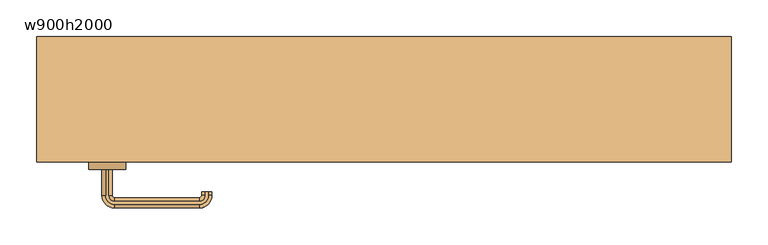
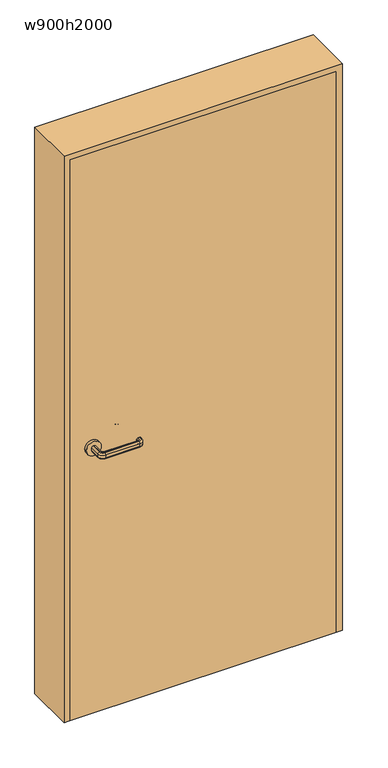
"""IFC4 building model written with IfcOpenShell, lengths in millimetres: door geometry, 片開き : w900h2000."""

from ifc_helpers import new_model, si_unit, point, frame, frame_2d, origin, origin_with_axes, place, context, project, spatial, polyline, circle_curve, ellipse_curve, trimmed, segment, composite_curve, outline, extrude, source, transform, mapped, element, save
from ifc_brep_helpers import plane_surface, cylinder_surface, revolved_surface, advanced_brep


def w900h2000_4bf1bc26(model_context):
    return source(origin(), model_context, "Body", "SolidModel", [
        advanced_brep(
        [(-377.0, -95.0, 960.0), (-373.0, -95.0, 960.0), (-368.0, -95.0, 955.0), (-368.0, -95.0, 945.0477623), (-373.0, -95.0, 940.0477623), (-377.0, -95.0, 940.0477623), (-382.0, -95.0, 945.0477623), (-382.0, -95.0, 955.0), (-382.0, -130.0, 955.0), (-377.0, -130.0, 960.0), (-382.0, -130.0, 945.0477623), (-377.0, -130.0, 940.0477623), (-373.0, -130.0, 940.0477623), (-365.0, -138.0, 940.0477623), (-250.0, -138.0, 940.0477623), (-242.0, -130.0, 940.0477623), (-242.0, -125.0, 940.0477623), (-238.0, -125.0, 940.0477623), (-238.0, -130.0, 940.0477623), (-250.0, -142.0, 940.0477623), (-365.0, -142.0, 940.0477623), (-368.0, -130.0, 945.0477623), (-368.0, -130.0, 955.0), (-373.0, -130.0, 960.0), (-365.0, -142.0, 960.0), (-250.0, -142.0, 960.0), (-238.0, -130.0, 960.0), (-238.0, -125.0, 960.0), (-242.0, -125.0, 960.0), (-242.0, -130.0, 960.0), (-250.0, -138.0, 960.0), (-365.0, -138.0, 960.0), (-365.0, -147.0, 955.0), (-365.0, -147.0, 945.0477623), (-365.0, -133.0, 945.0477623), (-365.0, -133.0, 955.0), (-250.0, -147.0, 955.0), (-250.0, -147.0, 945.0477623), (-250.0, -133.0, 945.0477623), (-250.0, -133.0, 955.0), (-233.0, -130.0, 955.0), (-233.0, -130.0, 945.0477623), (-247.0, -130.0, 945.0477623), (-247.0, -130.0, 955.0), (-233.0, -125.0, 955.0), (-233.0, -125.0, 945.0477623), (-247.0, -125.0, 945.0477623), (-247.0, -125.0, 955.0)],
        [
            (0, 1),
            (1, 2, circle_curve(frame((-373.0, -95.0, 955.0), z_axis=(0.0, 1.0, 0.0), x_axis=(-1.0, 0.0, 0.0)), 5.0)),
            (2, 3),
            (3, 4, circle_curve(frame((-373.0, -95.0, 945.0477623), z_axis=(0.0, 1.0, 0.0), x_axis=(-1.0, 0.0, 0.0)), 5.0)),
            (4, 5),
            (5, 6, circle_curve(frame((-377.0, -95.0, 945.0477623), z_axis=(0.0, 1.0, 0.0), x_axis=(-1.0, 0.0, 0.0)), 5.0)),
            (6, 7),
            (7, 0, circle_curve(frame((-377.0, -95.0, 955.0), z_axis=(0.0, 1.0, 0.0), x_axis=(-1.0, 0.0, 0.0)), 5.0)),
            (7, 8),
            (8, 9, circle_curve(frame((-377.0, -130.0, 955.0), z_axis=(0.0, 1.0, 0.0), x_axis=(-1.0, 0.0, 0.0)), 5.0)),
            (9, 0),
            (6, 10),
            (10, 8),
            (5, 11),
            (11, 10, circle_curve(frame((-377.0, -130.0, 945.0477623), z_axis=(0.0, 1.0, 0.0), x_axis=(-1.0, 0.0, 0.0)), 5.0)),
            (4, 12),
            (12, 13, circle_curve(frame((-365.0, -130.0, 940.0477623), z_axis=(0.0, 0.0, 1.0), x_axis=(-1.0, 0.0, 0.0)), 8.0)),
            (13, 14),
            (14, 15, circle_curve(frame((-250.0, -130.0, 940.0477623), z_axis=(0.0, 0.0, 1.0), x_axis=(0.0, -1.0, 0.0)), 8.0)),
            (15, 16),
            (16, 17),
            (17, 18),
            (18, 19, circle_curve(frame((-250.0, -130.0, 940.0477623), z_axis=(0.0, 0.0, -1.0), x_axis=(0.0, -1.0, 0.0)), 12.0)),
            (19, 20),
            (20, 11, circle_curve(frame((-365.0, -130.0, 940.0477623), z_axis=(0.0, 0.0, -1.0), x_axis=(-1.0, 0.0, 0.0)), 12.0)),
            (3, 21),
            (21, 12, circle_curve(frame((-373.0, -130.0, 945.0477623), z_axis=(0.0, 1.0, 0.0), x_axis=(-1.0, 0.0, 0.0)), 5.0)),
            (2, 22),
            (22, 21),
            (1, 23),
            (23, 22, circle_curve(frame((-373.0, -130.0, 955.0), z_axis=(0.0, 1.0, 0.0), x_axis=(-1.0, 0.0, 0.0)), 5.0)),
            (9, 24, circle_curve(frame((-365.0, -130.0, 960.0), z_axis=(0.0, 0.0, 1.0), x_axis=(-1.0, 0.0, 0.0)), 12.0)),
            (24, 25),
            (25, 26, circle_curve(frame((-250.0, -130.0, 960.0), z_axis=(0.0, 0.0, 1.0), x_axis=(0.0, -1.0, 0.0)), 12.0)),
            (26, 27),
            (27, 28),
            (28, 29),
            (29, 30, circle_curve(frame((-250.0, -130.0, 960.0), z_axis=(0.0, 0.0, -1.0), x_axis=(0.0, -1.0, 0.0)), 8.0)),
            (30, 31),
            (31, 23, circle_curve(frame((-365.0, -130.0, 960.0), z_axis=(0.0, 0.0, -1.0), x_axis=(-1.0, 0.0, 0.0)), 8.0)),
            (32, 24, circle_curve(frame((-365.0, -142.0, 955.0), z_axis=(-1.0, 0.0, 0.0), x_axis=(0.0, -1.0, 0.0)), 5.0)),
            (8, 32, circle_curve(frame((-365.0, -130.0, 955.0), z_axis=(0.0, 0.0, 1.0), x_axis=(-1.0, 0.0, 0.0)), 17.0)),
            (33, 32),
            (10, 33, circle_curve(frame((-365.0, -130.0, 945.0477623), z_axis=(0.0, 0.0, 1.0), x_axis=(-1.0, 0.0, 0.0)), 17.0)),
            (20, 33, circle_curve(frame((-365.0, -142.0, 945.0477623), z_axis=(-1.0, 0.0, 0.0), x_axis=(0.0, -1.0, 0.0)), 5.0)),
            (34, 13, circle_curve(frame((-365.0, -138.0, 945.0477623), z_axis=(-1.0, 0.0, 0.0), x_axis=(0.0, -1.0, 0.0)), 5.0)),
            (21, 34, circle_curve(frame((-365.0, -130.0, 945.0477623), z_axis=(0.0, 0.0, 1.0), x_axis=(-1.0, 0.0, 0.0)), 3.0)),
            (35, 34),
            (22, 35, circle_curve(frame((-365.0, -130.0, 955.0), z_axis=(0.0, 0.0, 1.0), x_axis=(-1.0, 0.0, 0.0)), 3.0)),
            (31, 35, circle_curve(frame((-365.0, -138.0, 955.0), z_axis=(-1.0, 0.0, 0.0), x_axis=(0.0, -1.0, 0.0)), 5.0)),
            (32, 36),
            (36, 25, circle_curve(frame((-250.0, -142.0, 955.0), z_axis=(-1.0, 0.0, 0.0), x_axis=(0.0, -1.0, 0.0)), 5.0)),
            (33, 37),
            (37, 36),
            (19, 37, circle_curve(frame((-250.0, -142.0, 945.0477623), z_axis=(-1.0, 0.0, 0.0), x_axis=(0.0, -1.0, 0.0)), 5.0)),
            (34, 38),
            (38, 14, circle_curve(frame((-250.0, -138.0, 945.0477623), z_axis=(-1.0, 0.0, 0.0), x_axis=(0.0, -1.0, 0.0)), 5.0)),
            (35, 39),
            (39, 38),
            (30, 39, circle_curve(frame((-250.0, -138.0, 955.0), z_axis=(-1.0, 0.0, 0.0), x_axis=(0.0, -1.0, 0.0)), 5.0)),
            (40, 26, circle_curve(frame((-238.0, -130.0, 955.0), z_axis=(0.0, -1.0, 0.0), x_axis=(1.0, 0.0, 0.0)), 5.0)),
            (36, 40, circle_curve(frame((-250.0, -130.0, 955.0), z_axis=(0.0, 0.0, 1.0), x_axis=(0.0, -1.0, 0.0)), 17.0)),
            (41, 40),
            (37, 41, circle_curve(frame((-250.0, -130.0, 945.0477623), z_axis=(0.0, 0.0, 1.0), x_axis=(0.0, -1.0, 0.0)), 17.0)),
            (18, 41, circle_curve(frame((-238.0, -130.0, 945.0477623), z_axis=(0.0, -1.0, 0.0), x_axis=(1.0, 0.0, 0.0)), 5.0)),
            (42, 15, circle_curve(frame((-242.0, -130.0, 945.0477623), z_axis=(0.0, -1.0, 0.0), x_axis=(1.0, 0.0, 0.0)), 5.0)),
            (38, 42, circle_curve(frame((-250.0, -130.0, 945.0477623), z_axis=(0.0, 0.0, 1.0), x_axis=(0.0, -1.0, 0.0)), 3.0)),
            (43, 42),
            (39, 43, circle_curve(frame((-250.0, -130.0, 955.0), z_axis=(0.0, 0.0, 1.0), x_axis=(0.0, -1.0, 0.0)), 3.0)),
            (29, 43, circle_curve(frame((-242.0, -130.0, 955.0), z_axis=(0.0, -1.0, 0.0), x_axis=(1.0, 0.0, 0.0)), 5.0)),
            (27, 44, circle_curve(frame((-238.0, -125.0, 955.0), z_axis=(0.0, 1.0, 0.0), x_axis=(1.0, 0.0, 0.0)), 5.0)),
            (44, 45),
            (45, 17, circle_curve(frame((-238.0, -125.0, 945.0477623), z_axis=(0.0, 1.0, 0.0), x_axis=(1.0, 0.0, 0.0)), 5.0)),
            (16, 46, circle_curve(frame((-242.0, -125.0, 945.0477623), z_axis=(0.0, 1.0, 0.0), x_axis=(1.0, 0.0, 0.0)), 5.0)),
            (46, 47),
            (47, 28, circle_curve(frame((-242.0, -125.0, 955.0), z_axis=(0.0, 1.0, 0.0), x_axis=(1.0, 0.0, 0.0)), 5.0)),
            (40, 44),
            (41, 45),
            (42, 46),
            (43, 47),
        ],
        [
            plane_surface(frame((-385.198039, -95.0, 950.0), z_axis=(0.0, 1.0, 0.0), x_axis=(0.0, 0.0, 1.0))),
            cylinder_surface(frame((-377.0, -95.0, 955.0), z_axis=(0.0, 1.0, 0.0), x_axis=(-1.0, 0.0, 0.0)), 5.0),
            plane_surface(frame((-382.0, -95.0, 955.0), z_axis=(-1.0, 0.0, 0.0), x_axis=(0.0, -1.0, 0.0))),
            cylinder_surface(frame((-377.0, -95.0, 945.0477623), z_axis=(0.0, 1.0, 0.0), x_axis=(-1.0, 0.0, 0.0)), 5.0),
            plane_surface(frame((-377.0, -95.0, 940.0477623), z_axis=(0.0, 0.0, -1.0), x_axis=(0.0, -1.0, 0.0))),
            cylinder_surface(frame((-373.0, -95.0, 945.0477623), z_axis=(0.0, 1.0, 0.0), x_axis=(-1.0, 0.0, 0.0)), 5.0),
            plane_surface(frame((-368.0, -95.0, 945.0477623), z_axis=(1.0, 0.0, 0.0), x_axis=(0.0, -1.0, 0.0))),
            cylinder_surface(frame((-373.0, -95.0, 955.0), z_axis=(0.0, 1.0, 0.0), x_axis=(-1.0, 0.0, 0.0)), 5.0),
            plane_surface(frame((-373.0, -95.0, 960.0), z_axis=(0.0, 0.0, 1.0), x_axis=(0.0, -1.0, 0.0))),
            revolved_surface(trimmed(ellipse_curve(frame((-377.0, -130.0, 955.0), z_axis=(0.0, -1.0, 0.0), x_axis=(-1.0, 0.0, 0.0)), 5.0, 5.0), [point((-377.0, -130.0, 960.0))], [point((-382.0, -130.0, 955.0))], True, "CARTESIAN"), (-365.0, -130.0, 950.0), (0.0, 0.0, -1.0)),
            cylinder_surface(frame((-365.0, -130.0, 950.0), z_axis=(0.0, 0.0, -1.0), x_axis=(-1.0, 0.0, 0.0)), 17.0),
            revolved_surface(trimmed(ellipse_curve(frame((-377.0, -130.0, 945.0477623), z_axis=(0.0, -1.0, 0.0), x_axis=(-1.0, 0.0, 0.0)), 5.0, 5.0), [point((-382.0, -130.0, 945.0477623))], [point((-377.0, -130.0, 940.0477623))], True, "CARTESIAN"), (-365.0, -130.0, 950.0), (0.0, 0.0, -1.0)),
            revolved_surface(trimmed(ellipse_curve(frame((-373.0, -130.0, 945.0477623), z_axis=(0.0, -1.0, 0.0), x_axis=(-1.0, 0.0, 0.0)), 5.0, 5.0), [point((-373.0, -130.0, 940.0477623))], [point((-368.0, -130.0, 945.0477623))], True, "CARTESIAN"), (-365.0, -130.0, 950.0), (0.0, 0.0, -1.0)),
            revolved_surface(polyline([(-368.0, -130.0, 945.0477623), (-368.0, -130.0, 955.0)]), (-365.0, -130.0, 950.0), (0.0, 0.0, -1.0)),
            revolved_surface(trimmed(ellipse_curve(frame((-373.0, -130.0, 955.0), z_axis=(0.0, -1.0, 0.0), x_axis=(-1.0, 0.0, 0.0)), 5.0, 5.0), [point((-368.0, -130.0, 955.0))], [point((-373.0, -130.0, 960.0))], True, "CARTESIAN"), (-365.0, -130.0, 950.0), (0.0, 0.0, -1.0)),
            cylinder_surface(frame((-365.0, -142.0, 955.0), z_axis=(-1.0, 0.0, 0.0), x_axis=(0.0, -1.0, 0.0)), 5.0),
            plane_surface(frame((-365.0, -147.0, 955.0), z_axis=(0.0, -1.0, 0.0), x_axis=(1.0, 0.0, 0.0))),
            cylinder_surface(frame((-365.0, -142.0, 945.0477623), z_axis=(-1.0, 0.0, 0.0), x_axis=(0.0, -1.0, 0.0)), 5.0),
            cylinder_surface(frame((-365.0, -138.0, 945.0477623), z_axis=(-1.0, 0.0, 0.0), x_axis=(0.0, -1.0, 0.0)), 5.0),
            plane_surface(frame((-365.0, -133.0, 945.0477623), z_axis=(0.0, 1.0, 0.0), x_axis=(1.0, 0.0, 0.0))),
            cylinder_surface(frame((-365.0, -138.0, 955.0), z_axis=(-1.0, 0.0, 0.0), x_axis=(0.0, -1.0, 0.0)), 5.0),
            revolved_surface(trimmed(ellipse_curve(frame((-250.0, -142.0, 955.0), z_axis=(1.0, 0.0, 0.0), x_axis=(0.0, -1.0, 0.0)), 5.0, 5.0), [point((-250.0, -142.0, 960.0))], [point((-250.0, -147.0, 955.0))], True, "CARTESIAN"), (-250.0, -130.0, 950.0), (0.0, 0.0, -1.0)),
            cylinder_surface(frame((-250.0, -130.0, 950.0), z_axis=(0.0, 0.0, -1.0), x_axis=(0.0, -1.0, 0.0)), 17.0),
            revolved_surface(trimmed(ellipse_curve(frame((-250.0, -142.0, 945.0477623), z_axis=(1.0, 0.0, 0.0), x_axis=(0.0, -1.0, 0.0)), 5.0, 5.0), [point((-250.0, -147.0, 945.0477623))], [point((-250.0, -142.0, 940.0477623))], True, "CARTESIAN"), (-250.0, -130.0, 950.0), (0.0, 0.0, -1.0)),
            revolved_surface(trimmed(ellipse_curve(frame((-250.0, -138.0, 945.0477623), z_axis=(1.0, 0.0, 0.0), x_axis=(0.0, -1.0, 0.0)), 5.0, 5.0), [point((-250.0, -138.0, 940.0477623))], [point((-250.0, -133.0, 945.0477623))], True, "CARTESIAN"), (-250.0, -130.0, 950.0), (0.0, 0.0, -1.0)),
            revolved_surface(polyline([(-250.0, -133.0, 945.0477623), (-250.0, -133.0, 955.0)]), (-250.0, -130.0, 950.0), (0.0, 0.0, -1.0)),
            revolved_surface(trimmed(ellipse_curve(frame((-250.0, -138.0, 955.0), z_axis=(1.0, 0.0, 0.0), x_axis=(0.0, -1.0, 0.0)), 5.0, 5.0), [point((-250.0, -133.0, 955.0))], [point((-250.0, -138.0, 960.0))], True, "CARTESIAN"), (-250.0, -130.0, 950.0), (0.0, 0.0, -1.0)),
            plane_surface(frame((-250.198039, -125.0, 950.0), z_axis=(0.0, 1.0, 0.0), x_axis=(0.0, 0.0, -1.0))),
            cylinder_surface(frame((-238.0, -130.0, 955.0), z_axis=(0.0, -1.0, 0.0), x_axis=(1.0, 0.0, 0.0)), 5.0),
            plane_surface(frame((-233.0, -130.0, 955.0), z_axis=(1.0, 0.0, 0.0), x_axis=(0.0, 1.0, 0.0))),
            cylinder_surface(frame((-238.0, -130.0, 945.0477623), z_axis=(0.0, -1.0, 0.0), x_axis=(1.0, 0.0, 0.0)), 5.0),
            cylinder_surface(frame((-242.0, -130.0, 945.0477623), z_axis=(0.0, -1.0, 0.0), x_axis=(1.0, 0.0, 0.0)), 5.0),
            plane_surface(frame((-247.0, -130.0, 945.0477623), z_axis=(-1.0, 0.0, 0.0), x_axis=(0.0, 1.0, 0.0))),
            cylinder_surface(frame((-242.0, -130.0, 955.0), z_axis=(0.0, -1.0, 0.0), x_axis=(1.0, 0.0, 0.0)), 5.0),
        ],
        [
            (0, [[1, 2, 3, 4, 5, 6, 7, 8]]),
            (1, [[9, 10, 11, -8]]),
            (2, [[12, 13, -9, -7]]),
            (3, [[14, 15, -12, -6]]),
            (4, [[16, 17, 18, 19, 20, 21, 22, 23, 24, 25, -14, -5]]),
            (5, [[26, 27, -16, -4]]),
            (6, [[28, 29, -26, -3]]),
            (7, [[30, 31, -28, -2]]),
            (8, [[-11, 32, 33, 34, 35, 36, 37, 38, 39, 40, -30, -1]]),
            (9, [[41, -32, -10, 42]]),
            (10, [[43, -42, -13, 44]]),
            (11, [[45, -44, -15, -25]]),
            (12, [[46, -17, -27, 47]]),
            (13, [[48, -47, -29, 49]]),
            (14, [[50, -49, -31, -40]]),
            (15, [[51, 52, -33, -41]]),
            (16, [[53, 54, -51, -43]]),
            (17, [[-24, 55, -53, -45]]),
            (18, [[56, 57, -18, -46]]),
            (19, [[58, 59, -56, -48]]),
            (20, [[-39, 60, -58, -50]]),
            (21, [[61, -34, -52, 62]]),
            (22, [[63, -62, -54, 64]]),
            (23, [[65, -64, -55, -23]]),
            (24, [[66, -19, -57, 67]]),
            (25, [[68, -67, -59, 69]]),
            (26, [[70, -69, -60, -38]]),
            (27, [[71, 72, 73, -21, 74, 75, 76, -36]]),
            (28, [[77, -71, -35, -61]]),
            (29, [[78, -72, -77, -63]]),
            (30, [[-22, -73, -78, -65]]),
            (31, [[79, -74, -20, -66]]),
            (32, [[80, -75, -79, -68]]),
            (33, [[-37, -76, -80, -70]]),
        ],
    ),
        advanced_brep(
        [(-373.0, -50.0, 940.0), (-368.0, -50.0, 945.0), (-368.0, -50.0, 955.0), (-373.0, -50.0, 960.0), (-377.0, -50.0, 960.0), (-382.0, -50.0, 955.0), (-382.0, -50.0, 945.0), (-377.0, -50.0, 940.0), (-377.0, -15.0, 940.0), (-365.0, -3.0, 940.0), (-250.0, -3.0, 940.0), (-238.0, -15.0, 940.0), (-238.0, -20.0, 940.0), (-242.0, -20.0, 940.0), (-242.0, -15.0, 940.0), (-250.0, -7.0, 940.0), (-365.0, -7.0, 940.0), (-373.0, -15.0, 940.0), (-382.0, -15.0, 945.0), (-382.0, -15.0, 955.0), (-377.0, -15.0, 960.0), (-373.0, -15.0, 960.0), (-365.0, -7.0, 960.0), (-250.0, -7.0, 960.0), (-242.0, -15.0, 960.0), (-242.0, -20.0, 960.0), (-238.0, -20.0, 960.0), (-238.0, -15.0, 960.0), (-250.0, -3.0, 960.0), (-365.0, -3.0, 960.0), (-368.0, -15.0, 955.0), (-368.0, -15.0, 945.0), (-365.0, 2.0, 945.0), (-365.0, 2.0, 955.0), (-365.0, -12.0, 955.0), (-365.0, -12.0, 945.0), (-250.0, 2.0, 945.0), (-250.0, 2.0, 955.0), (-250.0, -12.0, 955.0), (-250.0, -12.0, 945.0), (-233.0, -15.0, 945.0), (-233.0, -15.0, 955.0), (-247.0, -15.0, 955.0), (-247.0, -15.0, 945.0), (-233.0, -20.0, 945.0), (-233.0, -20.0, 955.0), (-247.0, -20.0, 955.0), (-247.0, -20.0, 945.0)],
        [
            (0, 1, circle_curve(frame((-373.0, -50.0, 945.0), z_axis=(0.0, -1.0, 0.0), x_axis=(1.0, 0.0, 0.0)), 5.0)),
            (1, 2),
            (2, 3, circle_curve(frame((-373.0, -50.0, 955.0), z_axis=(0.0, -1.0, 0.0), x_axis=(1.0, 0.0, 0.0)), 5.0)),
            (3, 4),
            (4, 5, circle_curve(frame((-377.0, -50.0, 955.0), z_axis=(0.0, -1.0, 0.0), x_axis=(1.0, 0.0, 0.0)), 5.0)),
            (5, 6),
            (6, 7, circle_curve(frame((-377.0, -50.0, 945.0), z_axis=(0.0, -1.0, 0.0), x_axis=(1.0, 0.0, 0.0)), 5.0)),
            (7, 0),
            (7, 8),
            (8, 9, circle_curve(frame((-365.0, -15.0, 940.0), z_axis=(0.0, 0.0, -1.0), x_axis=(-1.0, 0.0, 0.0)), 12.0)),
            (9, 10),
            (10, 11, circle_curve(frame((-250.0, -15.0, 940.0), z_axis=(0.0, 0.0, -1.0), x_axis=(0.0, 1.0, 0.0)), 12.0)),
            (11, 12),
            (12, 13),
            (13, 14),
            (14, 15, circle_curve(frame((-250.0, -15.0, 940.0), z_axis=(0.0, 0.0, 1.0), x_axis=(0.0, 1.0, 0.0)), 8.0)),
            (15, 16),
            (16, 17, circle_curve(frame((-365.0, -15.0, 940.0), z_axis=(0.0, 0.0, 1.0), x_axis=(-1.0, 0.0, 0.0)), 8.0)),
            (17, 0),
            (6, 18),
            (18, 8, circle_curve(frame((-377.0, -15.0, 945.0), z_axis=(0.0, -1.0, 0.0), x_axis=(1.0, 0.0, 0.0)), 5.0)),
            (5, 19),
            (19, 18),
            (4, 20),
            (20, 19, circle_curve(frame((-377.0, -15.0, 955.0), z_axis=(0.0, -1.0, 0.0), x_axis=(1.0, 0.0, 0.0)), 5.0)),
            (3, 21),
            (21, 22, circle_curve(frame((-365.0, -15.0, 960.0), z_axis=(0.0, 0.0, -1.0), x_axis=(-1.0, 0.0, 0.0)), 8.0)),
            (22, 23),
            (23, 24, circle_curve(frame((-250.0, -15.0, 960.0), z_axis=(0.0, 0.0, -1.0), x_axis=(0.0, 1.0, 0.0)), 8.0)),
            (24, 25),
            (25, 26),
            (26, 27),
            (27, 28, circle_curve(frame((-250.0, -15.0, 960.0), z_axis=(0.0, 0.0, 1.0), x_axis=(0.0, 1.0, 0.0)), 12.0)),
            (28, 29),
            (29, 20, circle_curve(frame((-365.0, -15.0, 960.0), z_axis=(0.0, 0.0, 1.0), x_axis=(-1.0, 0.0, 0.0)), 12.0)),
            (2, 30),
            (30, 21, circle_curve(frame((-373.0, -15.0, 955.0), z_axis=(0.0, -1.0, 0.0), x_axis=(1.0, 0.0, 0.0)), 5.0)),
            (1, 31),
            (31, 30),
            (17, 31, circle_curve(frame((-373.0, -15.0, 945.0), z_axis=(0.0, -1.0, 0.0), x_axis=(1.0, 0.0, 0.0)), 5.0)),
            (32, 9, circle_curve(frame((-365.0, -3.0, 945.0), z_axis=(-1.0, 0.0, 0.0), x_axis=(0.0, -1.0, 0.0)), 5.0)),
            (18, 32, circle_curve(frame((-365.0, -15.0, 945.0), z_axis=(0.0, 0.0, -1.0), x_axis=(-1.0, 0.0, 0.0)), 17.0)),
            (33, 32),
            (19, 33, circle_curve(frame((-365.0, -15.0, 955.0), z_axis=(0.0, 0.0, -1.0), x_axis=(-1.0, 0.0, 0.0)), 17.0)),
            (29, 33, circle_curve(frame((-365.0, -3.0, 955.0), z_axis=(-1.0, 0.0, 0.0), x_axis=(0.0, -1.0, 0.0)), 5.0)),
            (34, 22, circle_curve(frame((-365.0, -7.0, 955.0), z_axis=(-1.0, 0.0, 0.0), x_axis=(0.0, -1.0, 0.0)), 5.0)),
            (30, 34, circle_curve(frame((-365.0, -15.0, 955.0), z_axis=(0.0, 0.0, -1.0), x_axis=(-1.0, 0.0, 0.0)), 3.0)),
            (35, 34),
            (31, 35, circle_curve(frame((-365.0, -15.0, 945.0), z_axis=(0.0, 0.0, -1.0), x_axis=(-1.0, 0.0, 0.0)), 3.0)),
            (16, 35, circle_curve(frame((-365.0, -7.0, 945.0), z_axis=(-1.0, 0.0, 0.0), x_axis=(0.0, -1.0, 0.0)), 5.0)),
            (32, 36),
            (36, 10, circle_curve(frame((-250.0, -3.0, 945.0), z_axis=(-1.0, 0.0, 0.0), x_axis=(0.0, -1.0, 0.0)), 5.0)),
            (33, 37),
            (37, 36),
            (28, 37, circle_curve(frame((-250.0, -3.0, 955.0), z_axis=(-1.0, 0.0, 0.0), x_axis=(0.0, -1.0, 0.0)), 5.0)),
            (34, 38),
            (38, 23, circle_curve(frame((-250.0, -7.0, 955.0), z_axis=(-1.0, 0.0, 0.0), x_axis=(0.0, -1.0, 0.0)), 5.0)),
            (35, 39),
            (39, 38),
            (15, 39, circle_curve(frame((-250.0, -7.0, 945.0), z_axis=(-1.0, 0.0, 0.0), x_axis=(0.0, -1.0, 0.0)), 5.0)),
            (40, 11, circle_curve(frame((-238.0, -15.0, 945.0), z_axis=(0.0, 1.0, 0.0), x_axis=(-1.0, 0.0, 0.0)), 5.0)),
            (36, 40, circle_curve(frame((-250.0, -15.0, 945.0), z_axis=(0.0, 0.0, -1.0), x_axis=(0.0, 1.0, 0.0)), 17.0)),
            (41, 40),
            (37, 41, circle_curve(frame((-250.0, -15.0, 955.0), z_axis=(0.0, 0.0, -1.0), x_axis=(0.0, 1.0, 0.0)), 17.0)),
            (27, 41, circle_curve(frame((-238.0, -15.0, 955.0), z_axis=(0.0, 1.0, 0.0), x_axis=(-1.0, 0.0, 0.0)), 5.0)),
            (42, 24, circle_curve(frame((-242.0, -15.0, 955.0), z_axis=(0.0, 1.0, 0.0), x_axis=(-1.0, 0.0, 0.0)), 5.0)),
            (38, 42, circle_curve(frame((-250.0, -15.0, 955.0), z_axis=(0.0, 0.0, -1.0), x_axis=(0.0, 1.0, 0.0)), 3.0)),
            (43, 42),
            (39, 43, circle_curve(frame((-250.0, -15.0, 945.0), z_axis=(0.0, 0.0, -1.0), x_axis=(0.0, 1.0, 0.0)), 3.0)),
            (14, 43, circle_curve(frame((-242.0, -15.0, 945.0), z_axis=(0.0, 1.0, 0.0), x_axis=(-1.0, 0.0, 0.0)), 5.0)),
            (12, 44, circle_curve(frame((-238.0, -20.0, 945.0), z_axis=(0.0, -1.0, 0.0), x_axis=(-1.0, 0.0, 0.0)), 5.0)),
            (44, 45),
            (45, 26, circle_curve(frame((-238.0, -20.0, 955.0), z_axis=(0.0, -1.0, 0.0), x_axis=(-1.0, 0.0, 0.0)), 5.0)),
            (25, 46, circle_curve(frame((-242.0, -20.0, 955.0), z_axis=(0.0, -1.0, 0.0), x_axis=(-1.0, 0.0, 0.0)), 5.0)),
            (46, 47),
            (47, 13, circle_curve(frame((-242.0, -20.0, 945.0), z_axis=(0.0, -1.0, 0.0), x_axis=(-1.0, 0.0, 0.0)), 5.0)),
            (40, 44),
            (41, 45),
            (42, 46),
            (43, 47),
        ],
        [
            plane_surface(frame((-385.198039, -50.0, 950.0), z_axis=(0.0, -1.0, 0.0), x_axis=(0.0, 0.0, -1.0))),
            plane_surface(frame((-373.0, -50.0, 940.0), z_axis=(0.0, 0.0, -1.0), x_axis=(0.0, 1.0, 0.0))),
            cylinder_surface(frame((-377.0, -50.0, 945.0), z_axis=(0.0, -1.0, 0.0), x_axis=(1.0, 0.0, 0.0)), 5.0),
            plane_surface(frame((-382.0, -50.0, 945.0), z_axis=(-1.0, 0.0, 0.0), x_axis=(0.0, 1.0, 0.0))),
            cylinder_surface(frame((-377.0, -50.0, 955.0), z_axis=(0.0, -1.0, 0.0), x_axis=(1.0, 0.0, 0.0)), 5.0),
            plane_surface(frame((-377.0, -50.0, 960.0), z_axis=(0.0, 0.0, 1.0), x_axis=(0.0, 1.0, 0.0))),
            cylinder_surface(frame((-373.0, -50.0, 955.0), z_axis=(0.0, -1.0, 0.0), x_axis=(1.0, 0.0, 0.0)), 5.0),
            plane_surface(frame((-368.0, -50.0, 955.0), z_axis=(1.0, 0.0, 0.0), x_axis=(0.0, 1.0, 0.0))),
            cylinder_surface(frame((-373.0, -50.0, 945.0), z_axis=(0.0, -1.0, 0.0), x_axis=(1.0, 0.0, 0.0)), 5.0),
            revolved_surface(trimmed(ellipse_curve(frame((-377.0, -15.0, 945.0), z_axis=(0.0, 1.0, 0.0), x_axis=(1.0, 0.0, 0.0)), 5.0, 5.0), [point((-377.0, -15.0, 940.0))], [point((-382.0, -15.0, 945.0))], True, "CARTESIAN"), (-365.0, -15.0, 950.0), (0.0, 0.0, 1.0)),
            cylinder_surface(frame((-365.0, -15.0, 950.0), z_axis=(0.0, 0.0, 1.0), x_axis=(-1.0, 0.0, 0.0)), 17.0),
            revolved_surface(trimmed(ellipse_curve(frame((-377.0, -15.0, 955.0), z_axis=(0.0, 1.0, 0.0), x_axis=(1.0, 0.0, 0.0)), 5.0, 5.0), [point((-382.0, -15.0, 955.0))], [point((-377.0, -15.0, 960.0))], True, "CARTESIAN"), (-365.0, -15.0, 950.0), (0.0, 0.0, 1.0)),
            revolved_surface(trimmed(ellipse_curve(frame((-373.0, -15.0, 955.0), z_axis=(0.0, 1.0, 0.0), x_axis=(1.0, 0.0, 0.0)), 5.0, 5.0), [point((-373.0, -15.0, 960.0))], [point((-368.0, -15.0, 955.0))], True, "CARTESIAN"), (-365.0, -15.0, 950.0), (0.0, 0.0, 1.0)),
            revolved_surface(polyline([(-368.0, -15.0, 955.0), (-368.0, -15.0, 945.0)]), (-365.0, -15.0, 950.0), (0.0, 0.0, 1.0)),
            revolved_surface(trimmed(ellipse_curve(frame((-373.0, -15.0, 945.0), z_axis=(0.0, 1.0, 0.0), x_axis=(1.0, 0.0, 0.0)), 5.0, 5.0), [point((-368.0, -15.0, 945.0))], [point((-373.0, -15.0, 940.0))], True, "CARTESIAN"), (-365.0, -15.0, 950.0), (0.0, 0.0, 1.0)),
            cylinder_surface(frame((-365.0, -3.0, 945.0), z_axis=(-1.0, 0.0, 0.0), x_axis=(0.0, -1.0, 0.0)), 5.0),
            plane_surface(frame((-365.0, 2.0, 945.0), z_axis=(0.0, 1.0, 0.0), x_axis=(1.0, 0.0, 0.0))),
            cylinder_surface(frame((-365.0, -3.0, 955.0), z_axis=(-1.0, 0.0, 0.0), x_axis=(0.0, -1.0, 0.0)), 5.0),
            cylinder_surface(frame((-365.0, -7.0, 955.0), z_axis=(-1.0, 0.0, 0.0), x_axis=(0.0, -1.0, 0.0)), 5.0),
            plane_surface(frame((-365.0, -12.0, 955.0), z_axis=(0.0, -1.0, 0.0), x_axis=(1.0, 0.0, 0.0))),
            cylinder_surface(frame((-365.0, -7.0, 945.0), z_axis=(-1.0, 0.0, 0.0), x_axis=(0.0, -1.0, 0.0)), 5.0),
            revolved_surface(trimmed(ellipse_curve(frame((-250.0, -3.0, 945.0), z_axis=(1.0, 0.0, 0.0), x_axis=(0.0, -1.0, 0.0)), 5.0, 5.0), [point((-250.0, -3.0, 940.0))], [point((-250.0, 2.0, 945.0))], True, "CARTESIAN"), (-250.0, -15.0, 950.0), (0.0, 0.0, 1.0)),
            cylinder_surface(frame((-250.0, -15.0, 950.0), z_axis=(0.0, 0.0, 1.0), x_axis=(0.0, 1.0, 0.0)), 17.0),
            revolved_surface(trimmed(ellipse_curve(frame((-250.0, -3.0, 955.0), z_axis=(1.0, 0.0, 0.0), x_axis=(0.0, -1.0, 0.0)), 5.0, 5.0), [point((-250.0, 2.0, 955.0))], [point((-250.0, -3.0, 960.0))], True, "CARTESIAN"), (-250.0, -15.0, 950.0), (0.0, 0.0, 1.0)),
            revolved_surface(trimmed(ellipse_curve(frame((-250.0, -7.0, 955.0), z_axis=(1.0, 0.0, 0.0), x_axis=(0.0, -1.0, 0.0)), 5.0, 5.0), [point((-250.0, -7.0, 960.0))], [point((-250.0, -12.0, 955.0))], True, "CARTESIAN"), (-250.0, -15.0, 950.0), (0.0, 0.0, 1.0)),
            revolved_surface(polyline([(-250.0, -12.0, 955.0), (-250.0, -12.0, 945.0)]), (-250.0, -15.0, 950.0), (0.0, 0.0, 1.0)),
            revolved_surface(trimmed(ellipse_curve(frame((-250.0, -7.0, 945.0), z_axis=(1.0, 0.0, 0.0), x_axis=(0.0, -1.0, 0.0)), 5.0, 5.0), [point((-250.0, -12.0, 945.0))], [point((-250.0, -7.0, 940.0))], True, "CARTESIAN"), (-250.0, -15.0, 950.0), (0.0, 0.0, 1.0)),
            plane_surface(frame((-250.198039, -20.0, 950.0), z_axis=(0.0, -1.0, 0.0), x_axis=(0.0, 0.0, 1.0))),
            cylinder_surface(frame((-238.0, -15.0, 945.0), z_axis=(0.0, 1.0, 0.0), x_axis=(-1.0, 0.0, 0.0)), 5.0),
            plane_surface(frame((-233.0, -15.0, 945.0), z_axis=(1.0, 0.0, 0.0), x_axis=(0.0, -1.0, 0.0))),
            cylinder_surface(frame((-238.0, -15.0, 955.0), z_axis=(0.0, 1.0, 0.0), x_axis=(-1.0, 0.0, 0.0)), 5.0),
            cylinder_surface(frame((-242.0, -15.0, 955.0), z_axis=(0.0, 1.0, 0.0), x_axis=(-1.0, 0.0, 0.0)), 5.0),
            plane_surface(frame((-247.0, -15.0, 955.0), z_axis=(-1.0, 0.0, 0.0), x_axis=(0.0, -1.0, 0.0))),
            cylinder_surface(frame((-242.0, -15.0, 945.0), z_axis=(0.0, 1.0, 0.0), x_axis=(-1.0, 0.0, 0.0)), 5.0),
        ],
        [
            (0, [[1, 2, 3, 4, 5, 6, 7, 8]]),
            (1, [[9, 10, 11, 12, 13, 14, 15, 16, 17, 18, 19, -8]]),
            (2, [[20, 21, -9, -7]]),
            (3, [[22, 23, -20, -6]]),
            (4, [[24, 25, -22, -5]]),
            (5, [[26, 27, 28, 29, 30, 31, 32, 33, 34, 35, -24, -4]]),
            (6, [[36, 37, -26, -3]]),
            (7, [[38, 39, -36, -2]]),
            (8, [[-19, 40, -38, -1]]),
            (9, [[41, -10, -21, 42]]),
            (10, [[43, -42, -23, 44]]),
            (11, [[45, -44, -25, -35]]),
            (12, [[46, -27, -37, 47]]),
            (13, [[48, -47, -39, 49]]),
            (14, [[50, -49, -40, -18]]),
            (15, [[51, 52, -11, -41]]),
            (16, [[53, 54, -51, -43]]),
            (17, [[-34, 55, -53, -45]]),
            (18, [[56, 57, -28, -46]]),
            (19, [[58, 59, -56, -48]]),
            (20, [[-17, 60, -58, -50]]),
            (21, [[61, -12, -52, 62]]),
            (22, [[63, -62, -54, 64]]),
            (23, [[65, -64, -55, -33]]),
            (24, [[66, -29, -57, 67]]),
            (25, [[68, -67, -59, 69]]),
            (26, [[70, -69, -60, -16]]),
            (27, [[-14, 71, 72, 73, -31, 74, 75, 76]]),
            (28, [[77, -71, -13, -61]]),
            (29, [[78, -72, -77, -63]]),
            (30, [[-32, -73, -78, -65]]),
            (31, [[79, -74, -30, -66]]),
            (32, [[80, -75, -79, -68]]),
            (33, [[-15, -76, -80, -70]]),
        ],
    ),
        extrude(outline(composite_curve([segment(trimmed(circle_curve(frame_2d((950.0, -375.0)), 25.0), [point((950.0, -400.0))], [point((950.0, -350.0))], False, "CARTESIAN"), True, "CONTINUOUS"), segment(trimmed(circle_curve(frame_2d((950.0, -375.0)), 25.0), [point((950.0, -350.0))], [point((950.0, -400.0))], False, "CARTESIAN"), True, "CONTINUOUS")], self_intersect=False)), frame((0.0, -95.0, 0.0), z_axis=(0.0, 1.0, 0.0), x_axis=(0.0, 0.0, 1.0)), (0.0, 0.0, 1.0), 10.0),
        extrude(outline(composite_curve([segment(trimmed(circle_curve(frame_2d((950.0, -375.0)), 25.0), [point((950.0, -400.0))], [point((950.0, -350.0))], False, "CARTESIAN"), True, "CONTINUOUS"), segment(trimmed(circle_curve(frame_2d((950.0, -375.0)), 25.0), [point((950.0, -350.0))], [point((950.0, -400.0))], False, "CARTESIAN"), True, "CONTINUOUS")], self_intersect=False)), frame((0.0, -60.0, 0.0), z_axis=(0.0, 1.0, 0.0), x_axis=(0.0, 0.0, 1.0)), (0.0, 0.0, 1.0), 10.0),
        extrude(outline(polyline([(2020.0, -470.0), (0.0, -470.0), (0.0, -450.0), (2000.0, -450.0), (2000.0, 450.0), (0.0, 450.0), (0.0, 470.0), (2020.0, 470.0), (2020.0, -470.0)])), frame((0.0, -85.0, 0.0), z_axis=(0.0, 1.0, 0.0), x_axis=(0.0, 0.0, 1.0)), (0.0, 0.0, 1.0), 170.0),
        extrude(outline(polyline([(450.0, -60.0), (450.0, -85.0), (-450.0, -85.0), (-450.0, -60.0), (450.0, -60.0)])), origin_with_axes(), (0.0, 0.0, 1.0), 2000.0),
    ])


if __name__ == "__main__":
    model = new_model("IFC4")
    model_context = context("Model", 3, world=origin())
    ifc_project = project(units=[si_unit("LENGTHUNIT", "METRE", prefix="MILLI")], contexts=[model_context])
    site = spatial("IfcSite", under=ifc_project)
    building = spatial("IfcBuilding", under=site)
    placement = place(None, origin())
    w900h2000_shape = w900h2000_4bf1bc26(model_context)
    element("IfcDoor", 1, ObjectType="片開き : w900h2000", at=placement, inside=building, context=model_context, shape_type="MappedRepresentation", body=[
        mapped(w900h2000_shape, transform((0.0, 0.0, 0.0), x_axis=(1.0, 0.0, 0.0), y_axis=(0.0, 1.0, 0.0), z_axis=(0.0, 0.0, 1.0))),
    ])
    save(model, "model.ifc")

# Revit data of these elements
# Project information
#   プロジェクト発行日 = "発行日"
#   プロジェクト ステータス = "プロジェクト ステータス"
#   クライアント名 = "オーナ"
#   計画地住所 = "ここにアドレスを入力"
#   プロジェクト名 = "プロジェクト名"
#   プロジェクト番号 = "0001"
# Type "片開き : w900h2000"
#   Construction Type Id = "MDOOR"
#   Analytic Construction = "メタル"
#   Type Mark = "48"
#   Operation = "片側開き戸右"
#   Keynote = "08110.P2"
#   Visual Light Transmittance = 0
#   Solar Heat Gain Coefficient = 0
#   Heat Transfer Coefficient (U) = 3.7021 W/(m²·K)
#   高さ(中心) = 1000 mm
#   Height = 2000 mm
#   Thickness = 25 mm
#   ドア枠見附 = 20 mm
#   Width = 900 mm
#   取手取付け高さ = 950 mm
#   ドア枠ちり = 10 mm
#   Function = 0
#   ドア枠 [instance default] = 塗装ホワイト
#   ドア把手 [instance default] = メタル-ステンレス
#   ドア [instance default] = 塗装ホワイト
#   Wall Closure = (empty or 0)
# Element 1 (IfcDoor, "片開き : w900h2000")
#   Materials on its faces: "メタル-ステンレス", "塗装ホワイト"
# Materials
#   "塗装ホワイト": class "ペイント", colour RGB 249 249 249, transparency 0, Cost = 0
#   "メタル-ステンレス": class "メタル", colour RGB 247 247 247, transparency 0, Cost = 0
